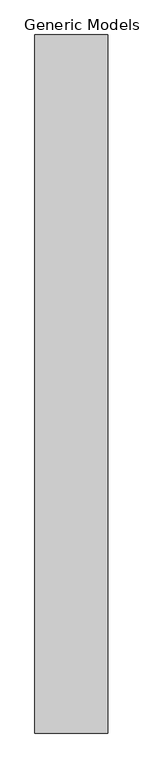
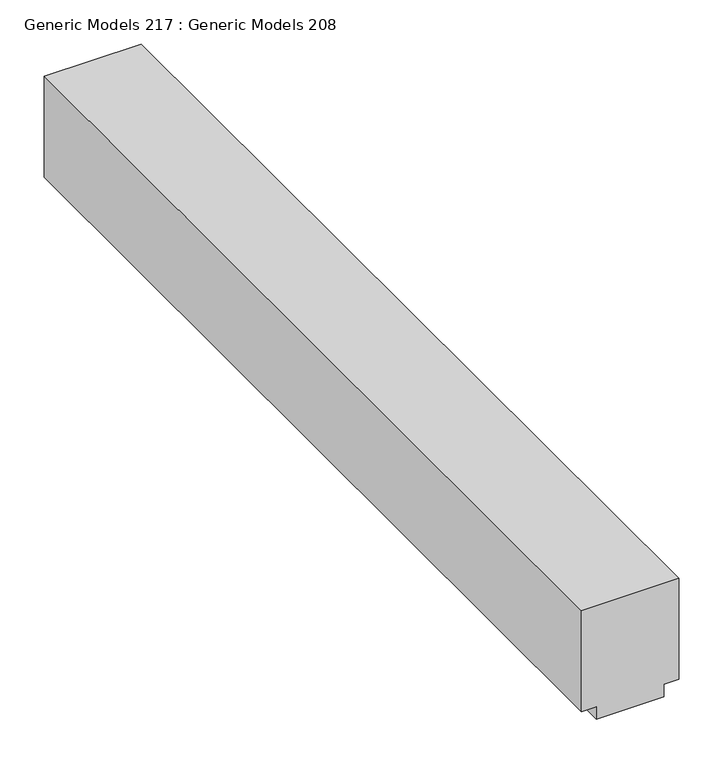
"""IFC4 building model written with IfcOpenShell, lengths in millimetres: proxy geometry, Generic Models 217 : Generic Models 208."""

from ifc_helpers import new_model, si_unit, frame, origin, place, context, project, spatial, polyline, outline, extrude, source, transform, mapped, element, save


def generic_models_217_generic_models_208_4c218d77(model_context):
    return source(origin(), model_context, "Body", "SweptSolid", [
        extrude(outline(polyline([(2188.765625, 55415.6329676), (2049.065625, 55415.6329676), (2049.065625, 55434.6829676), (2032.0, 55434.6829676), (2032.0, 55523.5829676), (2049.065625, 55523.5829676), (2049.065625, 55542.6329676), (2188.765625, 55542.6329676), (2188.765625, 55415.6329676)])), frame((0.0, -228.7033818, 0.0), z_axis=(0.0, 1.0, 0.0), x_axis=(0.0, 0.0, 1.0)), (0.0, 0.0, 1.0), 1219.2),
    ])


if __name__ == "__main__":
    model = new_model("IFC4")
    model_context = context("Model", 3, world=origin())
    ifc_project = project(units=[si_unit("LENGTHUNIT", "METRE", prefix="MILLI")], contexts=[model_context])
    site = spatial("IfcSite", under=ifc_project)
    building = spatial("IfcBuilding", under=site)
    placement = place(None, origin())
    generic_models_217_generic_models_208_shape = generic_models_217_generic_models_208_4c218d77(model_context)
    element("IfcBuildingElementProxy", 1, Name="Generic Models 217 : Generic Models 208", ObjectType="Generic Models 217 : Generic Models 208", at=placement, inside=building, context=model_context, shape_type="MappedRepresentation", body=[
        mapped(generic_models_217_generic_models_208_shape, transform((0.0, 0.0, 0.0), x_axis=(1.0, 0.0, 0.0), y_axis=(0.0, 1.0, 0.0), z_axis=(0.0, 0.0, 1.0))),
    ])
    save(model, "model.ifc")
